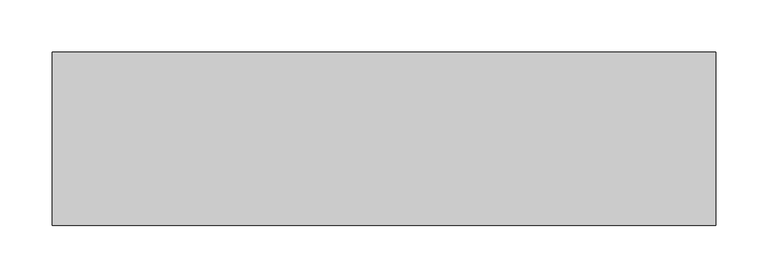
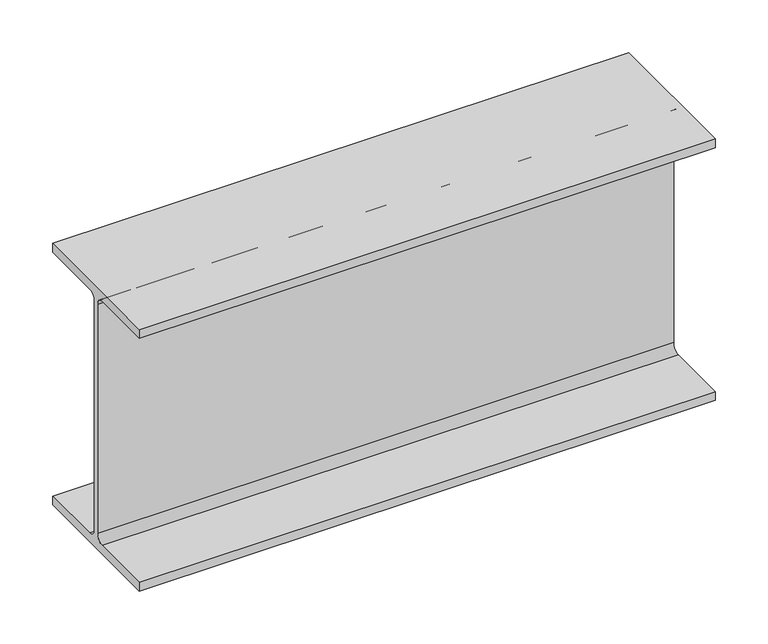
"""IFC4 building model written with IfcOpenShell, lengths in millimetres: beam geometry, Steel Beam_H-KSD3502 : H_SB_ASB_H-300x150x6.5x9."""

import ifcopenshell
import ifcopenshell.guid

model = None  # the IFC model being written
_history = None  # IfcOwnerHistory: only IFC2X3 demands one
_inside = {}  # id of a spatial element -> (the spatial element, [elements in it])
_under = {}  # id of a project, library or spatial element -> (it, [spatial elements below it])
_declared = {}  # id of a project -> (the project, [libraries it declares])
_typed = {}  # id of a type object -> (the type object, [elements of that type])
_made_of = {}  # id of a material, layer set ... -> (it, [elements and type objects made of it])


def new_model(schema):
    """Start an empty IFC model of exactly this schema.

    Asked for "IFC4X3", IfcOpenShell would pick the latest addendum, in which some entities
    have other attributes; the version numbers below select the first issue.
    IFC2X3 requires an IfcOwnerHistory on every rooted entity: one is made here for all.
    """
    global model, _history
    if schema == "IFC4X3":
        model = ifcopenshell.file(schema_version=(4, 3, 0, 0))
    else:
        model = ifcopenshell.file(schema=schema)
    _inside.clear()
    _under.clear()
    _declared.clear()
    _typed.clear()
    _made_of.clear()
    _history = None
    if model.schema == "IFC2X3":
        org = make("IfcOrganization", Name="unknown")
        user = make(
            "IfcPersonAndOrganization",
            ThePerson=make("IfcPerson", FamilyName="unknown"),
            TheOrganization=org,
        )
        app = make(
            "IfcApplication",
            ApplicationDeveloper=org,
            Version="unknown",
            ApplicationFullName="unknown",
            ApplicationIdentifier="unknown",
        )
        _history = make(
            "IfcOwnerHistory",
            OwningUser=user,
            OwningApplication=app,
            ChangeAction="ADDED",
            CreationDate=0,
        )
    return model


def make(cls, **values):
    """One entity of the class cls with the attributes given. An attribute that is None is left unset."""
    return model.create_entity(
        cls, **{name: value for name, value in values.items() if value is not None}
    )


def rooted(cls, **values):
    """An entity with a GlobalId (a new one), such as an element, a storey or a relation."""
    return make(cls, GlobalId=ifcopenshell.guid.new(), OwnerHistory=_history, **values)


def si_unit(unit_type, name, prefix=None):
    """IfcSIUnit, for example si_unit("LENGTHUNIT", "METRE", prefix="MILLI")."""
    return make("IfcSIUnit", UnitType=unit_type, Prefix=prefix, Name=name)


def assignment(units):
    """IfcUnitAssignment: the units of a project."""
    return None if units is None else make("IfcUnitAssignment", Units=units)


def point(xyz):
    """IfcCartesianPoint."""
    return None if xyz is None else make("IfcCartesianPoint", Coordinates=xyz)


def direction(xyz):
    """IfcDirection."""
    return None if xyz is None else make("IfcDirection", DirectionRatios=xyz)


def frame(location, z_axis=None, x_axis=None):
    """IfcAxis2Placement3D, a coordinate frame: its origin and axes. An axis left out is left unset."""
    return make(
        "IfcAxis2Placement3D",
        Location=point(location),
        Axis=direction(z_axis),
        RefDirection=direction(x_axis),
    )


def frame_2d(location, x_axis=None):
    """IfcAxis2Placement2D, a coordinate frame in the plane: its origin and x axis."""
    return make(
        "IfcAxis2Placement2D", Location=point(location), RefDirection=direction(x_axis)
    )


def origin():
    """The frame at (0, 0, 0) with its axes left unset."""
    return frame((0.0, 0.0, 0.0))


def place(relative_to, where):
    """IfcLocalPlacement: puts the frame where relative to a parent placement (None: the world)."""
    return make(
        "IfcLocalPlacement", PlacementRelTo=relative_to, RelativePlacement=where
    )


def context(
    kind, dimensions, precision=None, world=None, true_north=None, identifier=None
):
    """IfcGeometricRepresentationContext, for example the 3D "Model" context."""
    return make(
        "IfcGeometricRepresentationContext",
        ContextIdentifier=identifier,
        ContextType=kind,
        CoordinateSpaceDimension=dimensions,
        Precision=precision,
        WorldCoordinateSystem=world,
        TrueNorth=true_north,
    )


def project(units=None, contexts=None):
    """IfcProject with its units and contexts."""
    return rooted(
        "IfcProject",
        Name="project",
        RepresentationContexts=contexts,
        UnitsInContext=assignment(units),
    )


def spatial(cls, under=None, at=None, **own):
    """A site, building, storey or space (cls), placed at a placement, below another one or the project."""
    s = rooted(cls, ObjectPlacement=at, **own)
    if under is not None:
        _under.setdefault(under.id(), (under, []))[1].append(s)
    return s


def polyline(points):
    """IfcPolyline through the points."""
    return make("IfcPolyline", Points=[point(p) for p in points])


def circle_curve(where, radius):
    """IfcCircle in the frame where."""
    return make("IfcCircle", Position=where, Radius=radius)


def trimmed(basis, trim1, trim2, sense, master):
    """IfcTrimmedCurve: the piece of a basis curve between two trims."""
    return make(
        "IfcTrimmedCurve",
        BasisCurve=basis,
        Trim1=trim1,
        Trim2=trim2,
        SenseAgreement=sense,
        MasterRepresentation=master,
    )


def segment(curve, same_sense, transition):
    """IfcCompositeCurveSegment."""
    return make(
        "IfcCompositeCurveSegment",
        Transition=transition,
        SameSense=same_sense,
        ParentCurve=curve,
    )


def composite_curve(segments, self_intersect=None):
    """IfcCompositeCurve: segments joined end to end."""
    return make("IfcCompositeCurve", Segments=segments, SelfIntersect=self_intersect)


def outline(outer, holes=None, kind="AREA"):
    """IfcArbitraryClosedProfileDef: a profile drawn as a closed curve; with holes, ...WithVoids."""
    if holes is None:
        return make("IfcArbitraryClosedProfileDef", ProfileType=kind, OuterCurve=outer)
    return make(
        "IfcArbitraryProfileDefWithVoids",
        ProfileType=kind,
        OuterCurve=outer,
        InnerCurves=holes,
    )


def extrude(swept, where, along, depth):
    """IfcExtrudedAreaSolid: the profile swept, set in the frame where, extruded along a direction by depth."""
    return make(
        "IfcExtrudedAreaSolid",
        SweptArea=swept,
        Position=where,
        ExtrudedDirection=direction(along),
        Depth=depth,
    )


def shape(context_of_items, identifier, shape_type, items):
    """IfcShapeRepresentation: the items that make up one representation, for example the "Body"."""
    return make(
        "IfcShapeRepresentation",
        ContextOfItems=context_of_items,
        RepresentationIdentifier=identifier,
        RepresentationType=shape_type,
        Items=items,
    )


def source(mapping_origin, context_of_items, identifier, shape_type, items):
    """IfcRepresentationMap: a shape defined once, which mapped items show again and again."""
    return make(
        "IfcRepresentationMap",
        MappingOrigin=mapping_origin,
        MappedRepresentation=shape(context_of_items, identifier, shape_type, items),
    )


def transform(
    local_origin,
    x_axis=None,
    y_axis=None,
    z_axis=None,
    scale=None,
    scale2=None,
    scale3=None,
    uniform=True,
):
    """IfcCartesianTransformationOperator3D, or its non-uniform kind. x_axis, y_axis, z_axis: its Axis1, 2, 3."""
    if uniform:
        return make(
            "IfcCartesianTransformationOperator3D",
            Axis1=direction(x_axis),
            Axis2=direction(y_axis),
            LocalOrigin=point(local_origin),
            Scale=scale,
            Axis3=direction(z_axis),
        )
    return make(
        "IfcCartesianTransformationOperator3DnonUniform",
        Axis1=direction(x_axis),
        Axis2=direction(y_axis),
        LocalOrigin=point(local_origin),
        Scale=scale,
        Axis3=direction(z_axis),
        Scale2=scale2,
        Scale3=scale3,
    )


def mapped(mapping_source, mapping_target):
    """IfcMappedItem: shows the shape of a source again, moved by a transform."""
    return make(
        "IfcMappedItem", MappingSource=mapping_source, MappingTarget=mapping_target
    )


def made_of(thing, what):
    """Note that an element or type object is made of a material, layer set ...; save() writes the relation."""
    if what is not None:
        _made_of.setdefault(what.id(), (what, []))[1].append(thing)
    return thing


def element(
    cls,
    number,
    at=None,
    inside=None,
    cuts=None,
    type_object=None,
    material=None,
    context=None,
    identifier="Body",
    shape_type=None,
    held_by="IfcProductDefinitionShape",
    body=None,
    shapes=None,
    **own,
):
    """One element of the class cls, such as IfcWall. Its Tag is "e" and its number.

    at: its placement. inside: the storey or other place that contains it. cuts: it is an
    opening in that element (IfcRelVoidsElement). A single representation is given by context,
    identifier, shape_type and body (its items); several are given by shapes. held_by: the class
    of the entity that holds the representations. save() writes the other relations.
    """
    e = rooted(cls, Tag="e%d" % number, ObjectPlacement=at, **own)
    if body is not None:
        shapes = [shape(context, identifier, shape_type, body)]
    if shapes is not None:
        e.Representation = make(held_by, Representations=shapes)
    if inside is not None:
        _inside.setdefault(inside.id(), (inside, []))[1].append(e)
    if cuts is not None:
        rooted(
            "IfcRelVoidsElement", RelatingBuildingElement=cuts, RelatedOpeningElement=e
        )
    if type_object is not None:
        _typed.setdefault(type_object.id(), (type_object, []))[1].append(e)
    return made_of(e, material)


def aggregate(whole, parts):
    """IfcRelAggregates: a whole, such as a stair, and the parts it consists of."""
    return rooted("IfcRelAggregates", RelatingObject=whole, RelatedObjects=parts)


def save(model, path):
    """Write the relations noted so far, then the file.

    IfcRelAggregates (storeys below a building ...), IfcRelContainedInSpatialStructure (elements
    in a storey), IfcRelDefinesByType, IfcRelAssociatesMaterial and IfcRelDeclares: one each for
    every whole, place, type object, material and project.
    """
    for whole, parts in _under.values():
        aggregate(whole, parts)
    for where, things in _inside.values():
        rooted(
            "IfcRelContainedInSpatialStructure",
            RelatedElements=things,
            RelatingStructure=where,
        )
    for kind, things in _typed.values():
        rooted("IfcRelDefinesByType", RelatedObjects=things, RelatingType=kind)
    for what, things in _made_of.values():
        rooted("IfcRelAssociatesMaterial", RelatedObjects=things, RelatingMaterial=what)
    for by, libraries in _declared.values():
        rooted("IfcRelDeclares", RelatingContext=by, RelatedDefinitions=libraries)
    model.write(path)


def beam_96c0519e(model_context):
    return source(origin(), model_context, "Body", "SweptSolid", [
        extrude(outline(composite_curve([segment(polyline([(82.5, -141.5), (82.5, -151.7), (-82.5, -151.7), (-82.5, -141.5), (-11.9, -141.5)]), True, "CONTINUOUS"), segment(trimmed(circle_curve(frame_2d((-11.9, -132.6)), 8.9), [point((-11.9, -141.5))], [point((-3.0, -132.6))], True, "CARTESIAN"), True, "CONTINUOUS"), segment(polyline([(-3.0, -132.6), (-3.0, 132.6)]), True, "CONTINUOUS"), segment(trimmed(circle_curve(frame_2d((-11.9, 132.6)), 8.9), [point((-3.0, 132.6))], [point((-11.9, 141.5))], True, "CARTESIAN"), True, "CONTINUOUS"), segment(polyline([(-11.9, 141.5), (-82.5, 141.5), (-82.5, 151.7), (82.5, 151.7), (82.5, 141.5), (11.9, 141.5)]), True, "CONTINUOUS"), segment(trimmed(circle_curve(frame_2d((11.9, 132.6)), 8.9), [point((11.9, 141.5))], [point((3.0, 132.6))], True, "CARTESIAN"), True, "CONTINUOUS"), segment(polyline([(3.0, 132.6), (3.0, -132.6)]), True, "CONTINUOUS"), segment(trimmed(circle_curve(frame_2d((11.9, -132.6)), 8.9), [point((3.0, -132.6))], [point((11.9, -141.5))], True, "CARTESIAN"), True, "CONTINUOUS"), segment(polyline([(11.9, -141.5), (82.5, -141.5)]), True, "CONTINUOUS")], self_intersect=False)), frame((-238.55, 0.0, 0.0), z_axis=(1.0, 0.0, 0.0), x_axis=(0.0, 1.0, 0.0)), (0.0, 0.0, 1.0), 632.1),
    ])


if __name__ == "__main__":
    model = new_model("IFC4")
    model_context = context("Model", 3, world=origin())
    ifc_project = project(units=[si_unit("LENGTHUNIT", "METRE", prefix="MILLI")], contexts=[model_context])
    site = spatial("IfcSite", under=ifc_project)
    building = spatial("IfcBuilding", under=site)
    placement = place(None, origin())
    beam_shape = beam_96c0519e(model_context)
    element("IfcBeam", 1, ObjectType="Steel Beam_H-KSD3502 : H_SB_ASB_H-300x150x6.5x9", at=placement, inside=building, context=model_context, shape_type="MappedRepresentation", body=[
        mapped(beam_shape, transform((0.0, 0.0, 0.0), x_axis=(1.0, 0.0, 0.0), y_axis=(0.0, 1.0, 0.0), z_axis=(0.0, 0.0, 1.0))),
    ])
    save(model, "model.ifc")

# Revit data of these elements
# Type "Steel Beam_H-KSD3502 : H_SB_ASB_H-300x150x6.5x9"
#   Width = 15.0 cm
#   Web Thickness = 0.65 cm
#   Web Fillet = 1.3 cm
#   Warping Constant = 107174.0 cm⁶
#   Torsional Moment of Inertia = 9.9539 cm⁴
#   Torsional Modulus = 1.0 cm³
#   Section Area = 46.78 cm²
#   Plastic Modulus weak axis = 105.0 cm³
#   Plastic Modulus strong axis = 542.0 cm³
#   Perimeter = 1.17 m²/m
#   Nominal Weight = 36.70 kgf/m
#   Moment of Inertia weak axis = 508.00 cm⁴
#   Moment of Inertia strong axis = 7210.00 cm⁴
#   Height = 30.0 cm
#   Flange Thickness = 0.9 cm
#   Elastic Modulus weak axis = 67.7 cm³
#   Elastic Modulus strong axis = 481.0 cm³
#   Centroid Vertical = 15.0 cm
#   Centroid Horizontal = 7.5 cm
#   Length [instance default] = 1.5240 m
#   Structural Material [instance default] = Steel, 45-345
#   Assembly Code = ""
# Element 1 (IfcBeam, "Steel Beam_H-KSD3502 : H_SB_ASB_H-300x150x6.5x9")
#   Structural Material = none
# Materials
#   "Steel, 45-345": class "Metal", colour RGB 189 187 185, transparency 0, Description = "Steel 345 MPa", Cost = 0
